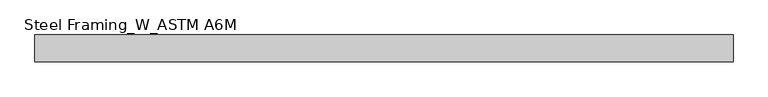
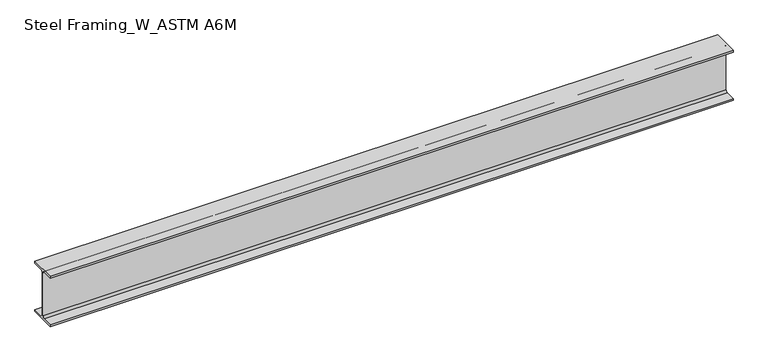
"""IFC4 building model written with IfcOpenShell, lengths in millimetres: beam geometry, Steel Framing_W_ASTM A6M : H_SB_AR_S02_W200x22.5_J1."""

from ifc_helpers import new_model, si_unit, point, frame, frame_2d, origin, place, context, project, spatial, polyline, circle_curve, trimmed, segment, composite_curve, outline, extrude, source, transform, mapped, element, save


def steel_framing_w_astm_a6m_d2b621d1(model_context):
    return source(origin(), model_context, "Body", "SweptSolid", [
        extrude(outline(composite_curve([segment(polyline([(51.0, -95.0), (51.0, -103.0), (-51.0, -103.0), (-51.0, -95.0), (-10.71, -95.0)]), True, "CONTINUOUS"), segment(trimmed(circle_curve(frame_2d((-10.71, -87.4)), 7.6), [point((-10.71, -95.0))], [point((-3.11, -87.4))], True, "CARTESIAN"), True, "CONTINUOUS"), segment(polyline([(-3.11, -87.4), (-3.11, 87.4)]), True, "CONTINUOUS"), segment(trimmed(circle_curve(frame_2d((-10.71, 87.4)), 7.6), [point((-3.11, 87.4))], [point((-10.71, 95.0))], True, "CARTESIAN"), True, "CONTINUOUS"), segment(polyline([(-10.71, 95.0), (-51.0, 95.0), (-51.0, 103.0), (51.0, 103.0), (51.0, 95.0), (10.71, 95.0)]), True, "CONTINUOUS"), segment(trimmed(circle_curve(frame_2d((10.71, 87.4)), 7.6), [point((10.71, 95.0))], [point((3.11, 87.4))], True, "CARTESIAN"), True, "CONTINUOUS"), segment(polyline([(3.11, 87.4), (3.11, -87.4)]), True, "CONTINUOUS"), segment(trimmed(circle_curve(frame_2d((10.71, -87.4)), 7.6), [point((3.11, -87.4))], [point((10.71, -95.0))], True, "CARTESIAN"), True, "CONTINUOUS"), segment(polyline([(10.71, -95.0), (51.0, -95.0)]), True, "CONTINUOUS")], self_intersect=False)), frame((-1319.7, 0.0, 0.0), z_axis=(1.0, 0.0, 0.0), x_axis=(0.0, 1.0, 0.0)), (0.0, 0.0, 1.0), 2639.4),
    ])


if __name__ == "__main__":
    model = new_model("IFC4")
    model_context = context("Model", 3, world=origin())
    ifc_project = project(units=[si_unit("LENGTHUNIT", "METRE", prefix="MILLI")], contexts=[model_context])
    site = spatial("IfcSite", under=ifc_project)
    building = spatial("IfcBuilding", under=site)
    placement = place(None, origin())
    steel_framing_w_astm_a6m_shape = steel_framing_w_astm_a6m_d2b621d1(model_context)
    element("IfcBeam", 1, ObjectType="Steel Framing_W_ASTM A6M : H_SB_AR_S02_W200x22.5_J1", at=placement, inside=building, context=model_context, shape_type="MappedRepresentation", body=[
        mapped(steel_framing_w_astm_a6m_shape, transform((0.0, 0.0, 0.0), x_axis=(1.0, 0.0, 0.0), y_axis=(0.0, 1.0, 0.0), z_axis=(0.0, 0.0, 1.0))),
    ])
    save(model, "model.ifc")

# Revit data of these elements
# Type "Steel Framing_W_ASTM A6M : H_SB_AR_S02_W200x22.5_J1"
#   Section Name Key = "W8x15"
#   Width = 10.2 cm
#   Web Thickness = 0.622 cm
#   Web Fillet = 0.76 cm
#   Warping Constant = 13900.0 cm⁶
#   Torsional Moment of Inertia = 5.70 cm⁴
#   Section Area = 28.6 cm²
#   Plastic Modulus weak axis = 43.8 cm³
#   Plastic Modulus strong axis = 223.0 cm³
#   Perimeter = 0.795 m²/m
#   Nominal Weight = 22.50 kgf/m
#   Moment of Inertia weak axis = 142.00 cm⁴
#   Moment of Inertia strong axis = 2000.00 cm⁴
#   Height = 20.6 cm
#   Flange Thickness = 0.8 cm
#   Elastic Modulus weak axis = 27.9 cm³
#   Elastic Modulus strong axis = 193.0 cm³
#   Centroid Vertical = 10.3 cm
#   Centroid Horizontal = 5.1 cm
#   Length [instance default] = 1500 mm
#   Structural Material [instance default] = Steel, 45-345
#   Bolt Spacing = 0
#   Assembly Code = ""
# Element 1 (IfcBeam, "Steel Framing_W_ASTM A6M : H_SB_AR_S02_W200x22.5_J1")
#   Materials on its faces: "Steel, 45-345"
# Materials
#   "Steel, 45-345": class "Metal", colour RGB 189 187 185, transparency 0, Description = "Steel 345 MPa", Cost = 0
